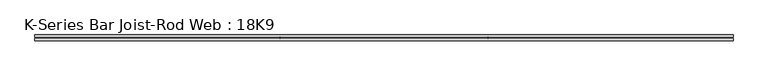
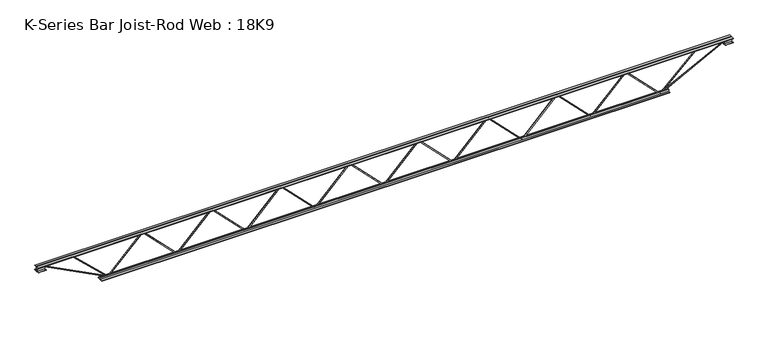
"""IFC4 building model written with IfcOpenShell, lengths in millimetres: beam geometry, K-Series Bar Joist-Rod Web : 18K9."""

import ifcopenshell
import ifcopenshell.guid

model = None  # the IFC model being written
_history = None  # IfcOwnerHistory: only IFC2X3 demands one
_inside = {}  # id of a spatial element -> (the spatial element, [elements in it])
_under = {}  # id of a project, library or spatial element -> (it, [spatial elements below it])
_declared = {}  # id of a project -> (the project, [libraries it declares])
_typed = {}  # id of a type object -> (the type object, [elements of that type])
_made_of = {}  # id of a material, layer set ... -> (it, [elements and type objects made of it])


def new_model(schema):
    """Start an empty IFC model of exactly this schema.

    Asked for "IFC4X3", IfcOpenShell would pick the latest addendum, in which some entities
    have other attributes; the version numbers below select the first issue.
    IFC2X3 requires an IfcOwnerHistory on every rooted entity: one is made here for all.
    """
    global model, _history
    if schema == "IFC4X3":
        model = ifcopenshell.file(schema_version=(4, 3, 0, 0))
    else:
        model = ifcopenshell.file(schema=schema)
    _inside.clear()
    _under.clear()
    _declared.clear()
    _typed.clear()
    _made_of.clear()
    _history = None
    if model.schema == "IFC2X3":
        org = make("IfcOrganization", Name="unknown")
        user = make(
            "IfcPersonAndOrganization",
            ThePerson=make("IfcPerson", FamilyName="unknown"),
            TheOrganization=org,
        )
        app = make(
            "IfcApplication",
            ApplicationDeveloper=org,
            Version="unknown",
            ApplicationFullName="unknown",
            ApplicationIdentifier="unknown",
        )
        _history = make(
            "IfcOwnerHistory",
            OwningUser=user,
            OwningApplication=app,
            ChangeAction="ADDED",
            CreationDate=0,
        )
    return model


def make(cls, **values):
    """One entity of the class cls with the attributes given. An attribute that is None is left unset."""
    return model.create_entity(
        cls, **{name: value for name, value in values.items() if value is not None}
    )


def rooted(cls, **values):
    """An entity with a GlobalId (a new one), such as an element, a storey or a relation."""
    return make(cls, GlobalId=ifcopenshell.guid.new(), OwnerHistory=_history, **values)


def si_unit(unit_type, name, prefix=None):
    """IfcSIUnit, for example si_unit("LENGTHUNIT", "METRE", prefix="MILLI")."""
    return make("IfcSIUnit", UnitType=unit_type, Prefix=prefix, Name=name)


def assignment(units):
    """IfcUnitAssignment: the units of a project."""
    return None if units is None else make("IfcUnitAssignment", Units=units)


def point(xyz):
    """IfcCartesianPoint."""
    return None if xyz is None else make("IfcCartesianPoint", Coordinates=xyz)


def direction(xyz):
    """IfcDirection."""
    return None if xyz is None else make("IfcDirection", DirectionRatios=xyz)


def frame(location, z_axis=None, x_axis=None):
    """IfcAxis2Placement3D, a coordinate frame: its origin and axes. An axis left out is left unset."""
    return make(
        "IfcAxis2Placement3D",
        Location=point(location),
        Axis=direction(z_axis),
        RefDirection=direction(x_axis),
    )


def origin():
    """The frame at (0, 0, 0) with its axes left unset."""
    return frame((0.0, 0.0, 0.0))


def place(relative_to, where):
    """IfcLocalPlacement: puts the frame where relative to a parent placement (None: the world)."""
    return make(
        "IfcLocalPlacement", PlacementRelTo=relative_to, RelativePlacement=where
    )


def context(
    kind, dimensions, precision=None, world=None, true_north=None, identifier=None
):
    """IfcGeometricRepresentationContext, for example the 3D "Model" context."""
    return make(
        "IfcGeometricRepresentationContext",
        ContextIdentifier=identifier,
        ContextType=kind,
        CoordinateSpaceDimension=dimensions,
        Precision=precision,
        WorldCoordinateSystem=world,
        TrueNorth=true_north,
    )


def project(units=None, contexts=None):
    """IfcProject with its units and contexts."""
    return rooted(
        "IfcProject",
        Name="project",
        RepresentationContexts=contexts,
        UnitsInContext=assignment(units),
    )


def spatial(cls, under=None, at=None, **own):
    """A site, building, storey or space (cls), placed at a placement, below another one or the project."""
    s = rooted(cls, ObjectPlacement=at, **own)
    if under is not None:
        _under.setdefault(under.id(), (under, []))[1].append(s)
    return s


def polyline(points):
    """IfcPolyline through the points."""
    return make("IfcPolyline", Points=[point(p) for p in points])


def outline(outer, holes=None, kind="AREA"):
    """IfcArbitraryClosedProfileDef: a profile drawn as a closed curve; with holes, ...WithVoids."""
    if holes is None:
        return make("IfcArbitraryClosedProfileDef", ProfileType=kind, OuterCurve=outer)
    return make(
        "IfcArbitraryProfileDefWithVoids",
        ProfileType=kind,
        OuterCurve=outer,
        InnerCurves=holes,
    )


def extrude(swept, where, along, depth):
    """IfcExtrudedAreaSolid: the profile swept, set in the frame where, extruded along a direction by depth."""
    return make(
        "IfcExtrudedAreaSolid",
        SweptArea=swept,
        Position=where,
        ExtrudedDirection=direction(along),
        Depth=depth,
    )


def shape(context_of_items, identifier, shape_type, items):
    """IfcShapeRepresentation: the items that make up one representation, for example the "Body"."""
    return make(
        "IfcShapeRepresentation",
        ContextOfItems=context_of_items,
        RepresentationIdentifier=identifier,
        RepresentationType=shape_type,
        Items=items,
    )


def source(mapping_origin, context_of_items, identifier, shape_type, items):
    """IfcRepresentationMap: a shape defined once, which mapped items show again and again."""
    return make(
        "IfcRepresentationMap",
        MappingOrigin=mapping_origin,
        MappedRepresentation=shape(context_of_items, identifier, shape_type, items),
    )


def transform(
    local_origin,
    x_axis=None,
    y_axis=None,
    z_axis=None,
    scale=None,
    scale2=None,
    scale3=None,
    uniform=True,
):
    """IfcCartesianTransformationOperator3D, or its non-uniform kind. x_axis, y_axis, z_axis: its Axis1, 2, 3."""
    if uniform:
        return make(
            "IfcCartesianTransformationOperator3D",
            Axis1=direction(x_axis),
            Axis2=direction(y_axis),
            LocalOrigin=point(local_origin),
            Scale=scale,
            Axis3=direction(z_axis),
        )
    return make(
        "IfcCartesianTransformationOperator3DnonUniform",
        Axis1=direction(x_axis),
        Axis2=direction(y_axis),
        LocalOrigin=point(local_origin),
        Scale=scale,
        Axis3=direction(z_axis),
        Scale2=scale2,
        Scale3=scale3,
    )


def mapped(mapping_source, mapping_target):
    """IfcMappedItem: shows the shape of a source again, moved by a transform."""
    return make(
        "IfcMappedItem", MappingSource=mapping_source, MappingTarget=mapping_target
    )


def made_of(thing, what):
    """Note that an element or type object is made of a material, layer set ...; save() writes the relation."""
    if what is not None:
        _made_of.setdefault(what.id(), (what, []))[1].append(thing)
    return thing


def element(
    cls,
    number,
    at=None,
    inside=None,
    cuts=None,
    type_object=None,
    material=None,
    context=None,
    identifier="Body",
    shape_type=None,
    held_by="IfcProductDefinitionShape",
    body=None,
    shapes=None,
    **own,
):
    """One element of the class cls, such as IfcWall. Its Tag is "e" and its number.

    at: its placement. inside: the storey or other place that contains it. cuts: it is an
    opening in that element (IfcRelVoidsElement). A single representation is given by context,
    identifier, shape_type and body (its items); several are given by shapes. held_by: the class
    of the entity that holds the representations. save() writes the other relations.
    """
    e = rooted(cls, Tag="e%d" % number, ObjectPlacement=at, **own)
    if body is not None:
        shapes = [shape(context, identifier, shape_type, body)]
    if shapes is not None:
        e.Representation = make(held_by, Representations=shapes)
    if inside is not None:
        _inside.setdefault(inside.id(), (inside, []))[1].append(e)
    if cuts is not None:
        rooted(
            "IfcRelVoidsElement", RelatingBuildingElement=cuts, RelatedOpeningElement=e
        )
    if type_object is not None:
        _typed.setdefault(type_object.id(), (type_object, []))[1].append(e)
    return made_of(e, material)


def aggregate(whole, parts):
    """IfcRelAggregates: a whole, such as a stair, and the parts it consists of."""
    return rooted("IfcRelAggregates", RelatingObject=whole, RelatedObjects=parts)


def save(model, path):
    """Write the relations noted so far, then the file.

    IfcRelAggregates (storeys below a building ...), IfcRelContainedInSpatialStructure (elements
    in a storey), IfcRelDefinesByType, IfcRelAssociatesMaterial and IfcRelDeclares: one each for
    every whole, place, type object, material and project.
    """
    for whole, parts in _under.values():
        aggregate(whole, parts)
    for where, things in _inside.values():
        rooted(
            "IfcRelContainedInSpatialStructure",
            RelatedElements=things,
            RelatingStructure=where,
        )
    for kind, things in _typed.values():
        rooted("IfcRelDefinesByType", RelatedObjects=things, RelatingType=kind)
    for what, things in _made_of.values():
        rooted("IfcRelAssociatesMaterial", RelatedObjects=things, RelatingMaterial=what)
    for by, libraries in _declared.values():
        rooted("IfcRelDeclares", RelatingContext=by, RelatedDefinitions=libraries)
    model.write(path)


def k_series_bar_joist_rod_web_18k9_1a6bf3c2(model_context):
    return source(origin(), model_context, "Body", "SweptSolid", [
        extrude(outline(polyline([(-217.4875, 1770.459375), (-227.0125, 1770.459375), (-227.0125, 1775.6332018), (217.4875, 2211.8980456), (217.4875, 2214.2503919), (-227.0125, 2650.5152357), (-227.0125, 2655.6890625), (-217.4875, 2655.6890625), (-217.4875, 2654.5128893), (227.0125, 2218.2480456), (227.0125, 2207.9003919), (-217.4875, 1771.6355482), (-217.4875, 1770.459375)])), frame((0.0, -4.7625, 0.0), z_axis=(0.0, 1.0, 0.0), x_axis=(0.0, 0.0, 1.0)), (0.0, 0.0, 1.0), 9.525),
        extrude(outline(polyline([(-217.4875, 885.2296875), (-227.0125, 885.2296875), (-227.0125, 890.4035143), (217.4875, 1326.6683581), (217.4875, 1329.0207044), (-227.0125, 1765.2855482), (-227.0125, 1770.459375), (-217.4875, 1770.459375), (-217.4875, 1769.2832018), (227.0125, 1333.0183581), (227.0125, 1322.6707044), (-217.4875, 886.4058607), (-217.4875, 885.2296875)])), frame((0.0, -4.7625, 0.0), z_axis=(0.0, 1.0, 0.0), x_axis=(0.0, 0.0, 1.0)), (0.0, 0.0, 1.0), 9.525),
        extrude(outline(polyline([(-217.4875, 0.0), (-227.0125, 0.0), (-227.0125, 5.1738268), (217.4875, 441.4386706), (217.4875, 443.7910169), (-227.0125, 880.0558607), (-227.0125, 885.2296875), (-217.4875, 885.2296875), (-217.4875, 884.0535143), (227.0125, 447.7886706), (227.0125, 437.4410169), (-217.4875, 1.1761732), (-217.4875, 0.0)])), frame((0.0, -4.7625, 0.0), z_axis=(0.0, 1.0, 0.0), x_axis=(0.0, 0.0, 1.0)), (0.0, 0.0, 1.0), 9.525),
        extrude(outline(polyline([(-217.4875, -885.2296875), (-227.0125, -885.2296875), (-227.0125, -880.0558607), (217.4875, -443.7910169), (217.4875, -441.4386706), (-227.0125, -5.1738268), (-227.0125, 0.0), (-217.4875, 0.0), (-217.4875, -1.1761732), (227.0125, -437.4410169), (227.0125, -447.7886706), (-217.4875, -884.0535143), (-217.4875, -885.2296875)])), frame((0.0, -4.7625, 0.0), z_axis=(0.0, 1.0, 0.0), x_axis=(0.0, 0.0, 1.0)), (0.0, 0.0, 1.0), 9.525),
        extrude(outline(polyline([(-217.4875, -1770.459375), (-227.0125, -1770.459375), (-227.0125, -1765.2855482), (217.4875, -1329.0207044), (217.4875, -1326.6683581), (-227.0125, -890.4035143), (-227.0125, -885.2296875), (-217.4875, -885.2296875), (-217.4875, -886.4058607), (227.0125, -1322.6707044), (227.0125, -1333.0183581), (-217.4875, -1769.2832018), (-217.4875, -1770.459375)])), frame((0.0, -4.7625, 0.0), z_axis=(0.0, 1.0, 0.0), x_axis=(0.0, 0.0, 1.0)), (0.0, 0.0, 1.0), 9.525),
        extrude(outline(polyline([(-217.4875, -2655.6890625), (-227.0125, -2655.6890625), (-227.0125, -2650.5152357), (217.4875, -2214.2503919), (217.4875, -2211.8980456), (-227.0125, -1775.6332018), (-227.0125, -1770.459375), (-217.4875, -1770.459375), (-217.4875, -1771.6355482), (227.0125, -2207.9003919), (227.0125, -2218.2480456), (-217.4875, -2654.5128893), (-217.4875, -2655.6890625)])), frame((0.0, -4.7625, 0.0), z_axis=(0.0, 1.0, 0.0), x_axis=(0.0, 0.0, 1.0)), (0.0, 0.0, 1.0), 9.525),
        extrude(outline(polyline([(-217.4875, 2655.6890625), (-227.0125, 2655.6890625), (-227.0125, 2660.8628893), (217.4875, 3097.1277331), (217.4875, 3099.4800794), (-227.0125, 3535.7449232), (-227.0125, 3540.91875), (-217.4875, 3540.91875), (-217.4875, 3539.7425768), (227.0125, 3103.4777331), (227.0125, 3093.1300794), (-217.4875, 2656.8652357), (-217.4875, 2655.6890625)])), frame((0.0, -4.7625, 0.0), z_axis=(0.0, 1.0, 0.0), x_axis=(0.0, 0.0, 1.0)), (0.0, 0.0, 1.0), 9.525),
        extrude(outline(polyline([(-217.4875, -3540.91875), (-227.0125, -3540.91875), (-227.0125, -3535.7449232), (217.4875, -3099.4800794), (217.4875, -3097.1277331), (-227.0125, -2660.8628893), (-227.0125, -2655.6890625), (-217.4875, -2655.6890625), (-217.4875, -2656.8652357), (227.0125, -3093.1300794), (227.0125, -3103.4777331), (-217.4875, -3539.7425768), (-217.4875, -3540.91875)])), frame((0.0, -4.7625, 0.0), z_axis=(0.0, 1.0, 0.0), x_axis=(0.0, 0.0, 1.0)), (0.0, 0.0, 1.0), 9.525),
        extrude(outline(polyline([(4.7625, 228.6), (36.5125, 228.6), (36.5125, 222.25), (11.1125, 222.25), (11.1125, 196.85), (4.7625, 196.85), (4.7625, 228.6)])), frame((-4455.31875, 0.0, 0.0), z_axis=(1.0, 0.0, 0.0), x_axis=(0.0, 1.0, 0.0)), (0.0, 0.0, 1.0), 8910.6375),
        extrude(outline(polyline([(-4.7625, 228.6), (-4.7625, 196.85), (-11.1125, 196.85), (-11.1125, 222.25), (-36.5125, 222.25), (-36.5125, 228.6), (-4.7625, 228.6)])), frame((-4455.31875, 0.0, 0.0), z_axis=(1.0, 0.0, 0.0), x_axis=(0.0, 1.0, 0.0)), (0.0, 0.0, 1.0), 8910.6375),
        extrude(outline(polyline([(-4.7625, 165.1), (-36.5125, 165.1), (-36.5125, 171.45), (-11.1125, 171.45), (-11.1125, 196.85), (-4.7625, 196.85), (-4.7625, 165.1)])), frame((-4455.31875, 0.0, 0.0), z_axis=(1.0, 0.0, 0.0), x_axis=(0.0, 1.0, 0.0)), (0.0, 0.0, 1.0), 101.6),
        extrude(outline(polyline([(36.5125, 165.1), (4.7625, 165.1), (4.7625, 196.85), (11.1125, 196.85), (11.1125, 171.45), (36.5125, 171.45), (36.5125, 165.1)])), frame((-4455.31875, 0.0, 0.0), z_axis=(1.0, 0.0, 0.0), x_axis=(0.0, 1.0, 0.0)), (0.0, 0.0, 1.0), 101.6),
        extrude(outline(polyline([(4.7625, 165.1), (4.7625, 196.85), (11.1125, 196.85), (11.1125, 171.45), (36.5125, 171.45), (36.5125, 165.1), (4.7625, 165.1)])), frame((4353.71875, 0.0, 0.0), z_axis=(1.0, 0.0, 0.0), x_axis=(0.0, 1.0, 0.0)), (0.0, 0.0, 1.0), 101.6),
        extrude(outline(polyline([(-4.7625, 165.1), (-36.5125, 165.1), (-36.5125, 171.45), (-11.1125, 171.45), (-11.1125, 196.85), (-4.7625, 196.85), (-4.7625, 165.1)])), frame((4353.71875, 0.0, 0.0), z_axis=(1.0, 0.0, 0.0), x_axis=(0.0, 1.0, 0.0)), (0.0, 0.0, 1.0), 101.6),
        extrude(outline(polyline([(4.7625, -228.6), (4.7625, -196.85), (11.1125, -196.85), (11.1125, -222.25), (36.5125, -222.25), (36.5125, -228.6), (4.7625, -228.6)])), frame((-3642.51875, 0.0, 0.0), z_axis=(1.0, 0.0, 0.0), x_axis=(0.0, 1.0, 0.0)), (0.0, 0.0, 1.0), 7285.0375),
        extrude(outline(polyline([(-4.7625, -228.6), (-36.5125, -228.6), (-36.5125, -222.25), (-11.1125, -222.25), (-11.1125, -196.85), (-4.7625, -196.85), (-4.7625, -228.6)])), frame((-3642.51875, 0.0, 0.0), z_axis=(1.0, 0.0, 0.0), x_axis=(0.0, 1.0, 0.0)), (0.0, 0.0, 1.0), 7285.0375),
        extrude(outline(polyline([(0.0, -9.525), (0.0, 0.0), (914.4881902, 0.0), (914.4881902, -9.525), (0.0, -9.525)])), frame((-4355.901352, 4.7625, 192.6170749), z_axis=(0.45828913319472747, 0.0, 0.8888031674086369), x_axis=(0.8888031674086369, 0.0, -0.45828913319472747)), (0.0, 0.0, 1.0), 9.525),
        extrude(outline(polyline([(0.0, -9.525), (0.0, 0.0), (609.5512365, 0.0), (609.5512365, -9.525), (0.0, -9.525)])), frame((-3986.8080744, 4.7625, 193.3917949), z_axis=(0.6875549993342648, 0.0, 0.7261323039849275), x_axis=(0.7261323039849275, 0.0, -0.6875549993342648)), (0.0, 0.0, 1.0), 9.525),
        extrude(outline(polyline([(0.0, -9.525), (0.0, 0.0), (914.4881902, 0.0), (914.4881902, -9.525), (0.0, -9.525)])), frame((4355.901352, -4.7625, 192.6170749), z_axis=(-0.4582891331947154, 0.0, 0.8888031674086431), x_axis=(-0.8888031674086431, 0.0, -0.4582891331947154)), (0.0, 0.0, 1.0), 9.525),
        extrude(outline(polyline([(0.0, -9.525), (0.0, 0.0), (609.5512365, 0.0), (609.5512365, -9.525), (0.0, -9.525)])), frame((3986.8080744, -4.7625, 193.3917949), z_axis=(-0.6875549993342612, 0.0, 0.726132303984931), x_axis=(-0.726132303984931, 0.0, -0.6875549993342612)), (0.0, 0.0, 1.0), 9.525),
    ])


if __name__ == "__main__":
    model = new_model("IFC4")
    model_context = context("Model", 3, world=origin())
    ifc_project = project(units=[si_unit("LENGTHUNIT", "METRE", prefix="MILLI")], contexts=[model_context])
    site = spatial("IfcSite", under=ifc_project)
    building = spatial("IfcBuilding", under=site)
    placement = place(None, origin())
    k_series_bar_joist_rod_web_18k9_shape = k_series_bar_joist_rod_web_18k9_1a6bf3c2(model_context)
    element("IfcBeam", 1, ObjectType="K-Series Bar Joist-Rod Web : 18K9", at=placement, inside=building, context=model_context, shape_type="MappedRepresentation", body=[
        mapped(k_series_bar_joist_rod_web_18k9_shape, transform((0.0, 0.0, 0.0), x_axis=(1.0, 0.0, 0.0), y_axis=(0.0, 1.0, 0.0), z_axis=(0.0, 0.0, 1.0))),
    ])
    save(model, "model.ifc")

# Revit data of these elements
# Type "K-Series Bar Joist-Rod Web : 18K9"
#   Assembly Code = "B1010350"
#   Wt = 10.2
#   Web Thickness = 0' - 0 3/8"
#   Start Offset [instance default] = 0' - 0"
#   Start Extension [instance default] = 0' - 0"
#   Seat Length = 0' - 4"
#   Seat Depth = 0' - 2 1/2"
#   PanelArrayLength [instance default] = 18' - 0"
#   Panel [instance default] = 3' - 0"
#   End Offset [instance default] = 0' - 0"
#   End Extension [instance default] = 0' - 0"
#   End Panel = 3' - 0"
#   Cord Leg = 0' - 1 1/4"
#   Chord Thickness = 0' - 0 1/4"
#   Length [instance default] = 24' - 0"
#   Depth = 1' - 6"
#   PanelArrayNum [instance default] = 6
#   Structural Material = none
# Element 1 (IfcBeam, "K-Series Bar Joist-Rod Web : 18K9")
#   PanelArrayLength = 23' - 2 13/16"
#   Panel = 2' - 10 109/128"
#   PanelArrayNum = 8
